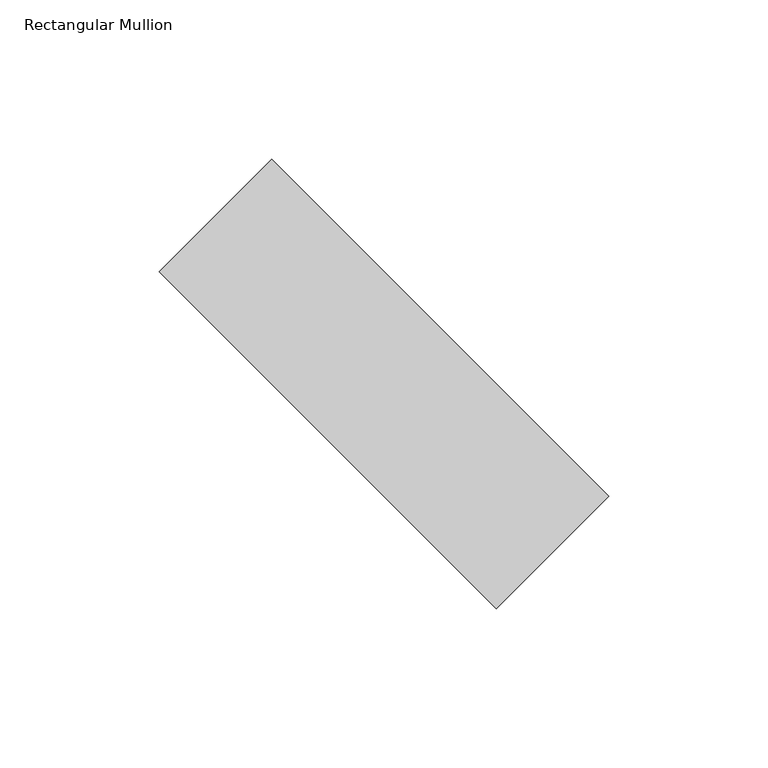
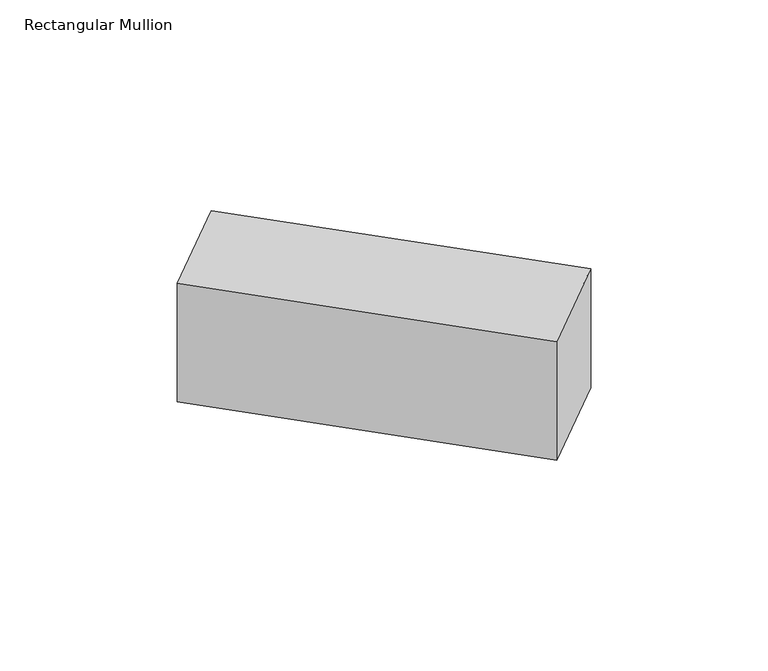
"""IFC4 building model written with IfcOpenShell, lengths in millimetres: member geometry, Rectangular Mullion : tilted mullions."""

from ifc_helpers import new_model, si_unit, frame, origin, place, context, project, spatial, polyline, outline, extrude, source, transform, mapped, element, save


def rectangular_mullion_ce6685f0(model_context):
    return source(origin(), model_context, "Body", "SweptSolid", [
        extrude(outline(polyline([(-35.3553391, 70.7106781), (70.7106781, -35.3553391), (35.3553391, -70.7106781), (-70.7106781, 35.3553391), (-35.3553391, 70.7106781)])), frame((0.0, 0.0, -55.2367034), z_axis=(0.0, 0.0, 1.0), x_axis=(1.0, 0.0, 0.0)), (0.0, 0.0, 1.0), 55.2367034),
    ])


if __name__ == "__main__":
    model = new_model("IFC4")
    model_context = context("Model", 3, world=origin())
    ifc_project = project(units=[si_unit("LENGTHUNIT", "METRE", prefix="MILLI")], contexts=[model_context])
    site = spatial("IfcSite", under=ifc_project)
    building = spatial("IfcBuilding", under=site)
    placement = place(None, origin())
    rectangular_mullion_shape = rectangular_mullion_ce6685f0(model_context)
    element("IfcMember", 1, ObjectType="Rectangular Mullion : tilted mullions", at=placement, inside=building, context=model_context, shape_type="MappedRepresentation", body=[
        mapped(rectangular_mullion_shape, transform((0.0, 0.0, 0.0), x_axis=(1.0, 0.0, 0.0), y_axis=(0.0, 1.0, 0.0), z_axis=(0.0, 0.0, 1.0))),
    ])
    save(model, "model.ifc")

# Revit data of these elements
# Type "Rectangular Mullion : tilted mullions"
#   built-in parameter 1007304 = 0.492126 (stored number, unit not read)
#   built-in parameter 1007301 = 0.082021 (stored number, unit not read)
#   built-in parameter 1007300 = 0.082021 (stored number, unit not read)
# Element 1 (IfcMember, "Rectangular Mullion : tilted mullions")
#   Materials on its faces: "Aluminum"
# Materials
#   "Aluminum": class "Metal", colour RGB 244 244 244, transparency 0, Description = "Aluminum 6061", Cost = 0
